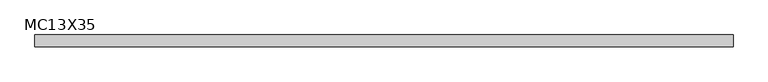
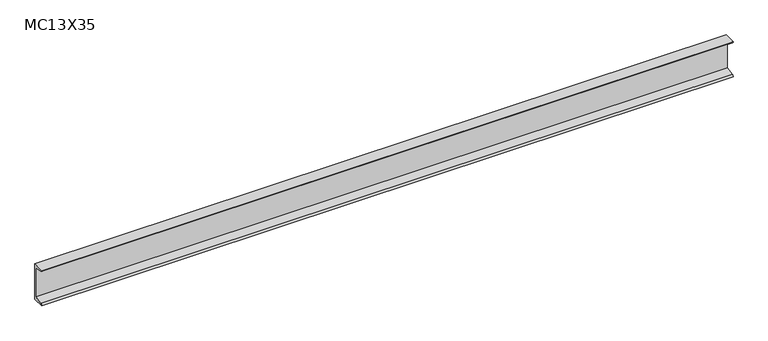
"""IFC4 building model written with IfcOpenShell, lengths in millimetres: beam geometry, MC-Miscellaneous Channel : MC13X35."""

from ifc_helpers import new_model, si_unit, point, frame, frame_2d, origin, place, context, project, spatial, polyline, circle_curve, trimmed, segment, composite_curve, outline, extrude, source, transform, mapped, element, save


def mc13x35_057ada5b(model_context):
    return source(origin(), model_context, "Body", "SweptSolid", [
        extrude(outline(composite_curve([segment(polyline([(24.892, 165.1), (24.892, -165.1), (-78.486, -165.1)]), True, "CONTINUOUS"), segment(trimmed(circle_curve(frame_2d((-62.992, -165.1)), 15.494), [point((-78.486, -165.1))], [point((-62.992, -149.606))], False, "CARTESIAN"), True, "CONTINUOUS"), segment(polyline([(-62.992, -149.606), (13.5382, -137.4848071), (13.5382, 137.4848071), (-62.992, 149.606)]), True, "CONTINUOUS"), segment(trimmed(circle_curve(frame_2d((-62.992, 165.1)), 15.494), [point((-62.992, 149.606))], [point((-78.486, 165.1))], False, "CARTESIAN"), True, "CONTINUOUS"), segment(polyline([(-78.486, 165.1), (24.892, 165.1)]), True, "CONTINUOUS")], self_intersect=False)), frame((-3035.3, 0.0, 0.0), z_axis=(1.0, 0.0, 0.0), x_axis=(0.0, 1.0, 0.0)), (0.0, 0.0, 1.0), 6146.7999994),
    ])


if __name__ == "__main__":
    model = new_model("IFC4")
    model_context = context("Model", 3, world=origin())
    ifc_project = project(units=[si_unit("LENGTHUNIT", "METRE", prefix="MILLI")], contexts=[model_context])
    site = spatial("IfcSite", under=ifc_project)
    building = spatial("IfcBuilding", under=site)
    placement = place(None, origin())
    mc13x35_shape = mc13x35_057ada5b(model_context)
    element("IfcBeam", 1, ObjectType="MC-Miscellaneous Channel : MC13X35", at=placement, inside=building, context=model_context, shape_type="MappedRepresentation", body=[
        mapped(mc13x35_shape, transform((0.0, 0.0, 0.0), x_axis=(1.0, 0.0, 0.0), y_axis=(0.0, 1.0, 0.0), z_axis=(0.0, 0.0, 1.0))),
    ])
    save(model, "model.ifc")

# Revit data of these elements
# Type "MC-Miscellaneous Channel : MC13X35"
#   Assembly Code = "B10"
#   W = 35
#   Length [instance default] = 5' - 0"
#   bf = 0' - 4.07"
#   d = 1' - 1"
#   tf = 0' - 0.61"
#   tw = 0' - 0.447"
#   x = 0' - 0.98"
#   A = 0.0715278 SF
#   Structural Material [instance default] = Steel ASTM A36
# Element 1 (IfcBeam, "MC-Miscellaneous Channel : MC13X35")
#   Materials on its faces: "Steel ASTM A36"
# Materials
#   "Steel ASTM A36": class "Metal", colour RGB 199 199 199, transparency 0, Description = "Structural steel, ASTM A36 Grade B, mill finish", Cost = 0
